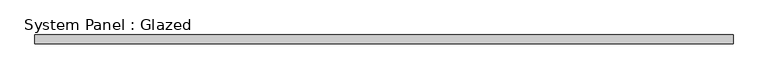
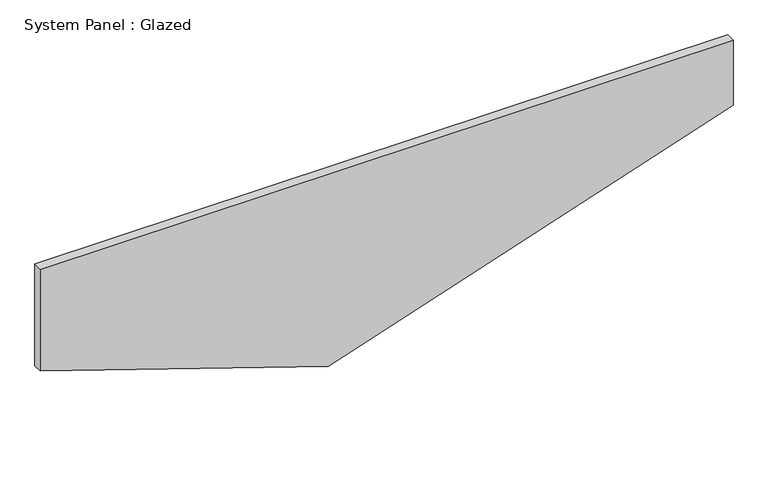
"""IFC4 building model written with IfcOpenShell, lengths in millimetres: plate geometry, System Panel : Glazed."""

from ifc_helpers import new_model, si_unit, frame, origin, place, context, project, spatial, polyline, outline, extrude, source, transform, mapped, element, save


def system_panel_glazed_6a6e56af(model_context):
    return source(origin(), model_context, "Body", "SweptSolid", [
        extrude(outline(polyline([(273.05, -984.25), (0.0, -165.1), (383.1166667, 984.25), (579.0943793, 984.25), (579.0943793, -984.25), (273.05, -984.25)])), frame((0.0, -44.45, 0.0), z_axis=(0.0, 1.0, 0.0), x_axis=(0.0, 0.0, 1.0)), (0.0, 0.0, 1.0), 25.4),
    ])


if __name__ == "__main__":
    model = new_model("IFC4")
    model_context = context("Model", 3, world=origin())
    ifc_project = project(units=[si_unit("LENGTHUNIT", "METRE", prefix="MILLI")], contexts=[model_context])
    site = spatial("IfcSite", under=ifc_project)
    building = spatial("IfcBuilding", under=site)
    placement = place(None, origin())
    system_panel_glazed_shape = system_panel_glazed_6a6e56af(model_context)
    element("IfcPlate", 1, ObjectType="System Panel : Glazed", at=placement, inside=building, context=model_context, shape_type="MappedRepresentation", body=[
        mapped(system_panel_glazed_shape, transform((0.0, 0.0, 0.0), x_axis=(1.0, 0.0, 0.0), y_axis=(0.0, 1.0, 0.0), z_axis=(0.0, 0.0, 1.0))),
    ])
    save(model, "model.ifc")

# Revit data of these elements
# Element 1 (IfcPlate, "System Panel : Glazed")
#   Materials on its faces: "Glass"
# Materials
#   "Glass": class "Glass", colour RGB 0 128 192, transparency 0.75
